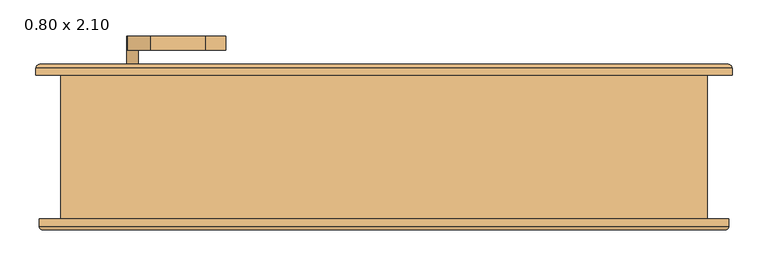
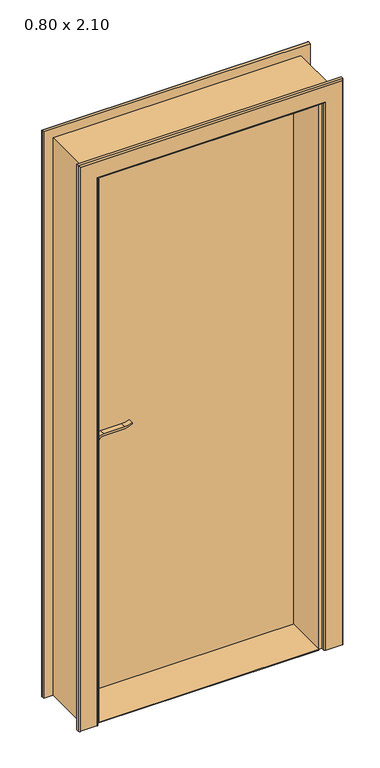
"""IFC4 building model written with IfcOpenShell, lengths in millimetres: door geometry, PORTA_DE_ABRIR_MADEIRA : 0.80 x 2.10."""

from ifc_helpers import new_model, si_unit, point, frame, frame_2d, origin, origin_with_axes, place, context, project, spatial, polyline, circle_curve, ellipse_curve, trimmed, segment, composite_curve, outline, extrude, faceted_brep, source, transform, mapped, element, save
from ifc_brep_helpers import plane_surface, cylinder_surface, advanced_brep


def door_0_80_x_2_10_3d2226a5(model_context):
    return source(origin(), model_context, "Body", "SolidModel", [
        extrude(outline(composite_curve([segment(trimmed(circle_curve(frame_2d((940.0, -350.0)), 15.0), [point((940.0, -335.0))], [point((940.0, -365.0))], False, "CARTESIAN"), True, "CONTINUOUS"), segment(trimmed(circle_curve(frame_2d((940.0, -350.0)), 15.0), [point((940.0, -365.0))], [point((940.0, -335.0))], False, "CARTESIAN"), True, "CONTINUOUS")], self_intersect=False)), frame((0.0, 40.0, 0.0), z_axis=(0.0, 1.0, 0.0), x_axis=(0.0, 0.0, 1.0)), (0.0, 0.0, 1.0), 10.0),
        extrude(outline(composite_curve([segment(trimmed(circle_curve(frame_2d((940.0, -350.0)), 15.0), [point((940.0, -335.0))], [point((940.0, -365.0))], False, "CARTESIAN"), True, "CONTINUOUS"), segment(trimmed(circle_curve(frame_2d((940.0, -350.0)), 15.0), [point((940.0, -365.0))], [point((940.0, -335.0))], False, "CARTESIAN"), True, "CONTINUOUS")], self_intersect=False)), frame((0.0, 105.0, 0.0), z_axis=(0.0, 1.0, 0.0), x_axis=(0.0, 0.0, 1.0)), (0.0, 0.0, 1.0), 10.0),
        extrude(outline(composite_curve([segment(trimmed(circle_curve(frame_2d((1000.0, -350.0)), 8.0), [point((1004.6523287, -356.5081363))], [point((1000.0, -342.0))], False, "CARTESIAN"), True, "CONTINUOUS"), segment(trimmed(circle_curve(frame_2d((994.8738613, -324.6138099)), 18.1261387), [point((1000.0, -342.0))], [point((1013.0, -324.6138099))], True, "CARTESIAN"), True, "CONTINUOUS"), segment(polyline([(1013.0, -324.6138099), (1013.0, -248.3564091)]), True, "CONTINUOUS"), segment(trimmed(circle_curve(frame_2d((1072.2709207, -251.9396612)), 59.3791355), [point((1013.0, -248.3564091))], [point((1022.2135558, -220.0))], False, "CARTESIAN"), True, "CONTINUOUS"), segment(polyline([(1022.2135558, -220.0), (1025.0, -220.0)]), True, "CONTINUOUS"), segment(trimmed(circle_curve(frame_2d((1103.2850638, -248.4227909)), 83.2850902), [point((1025.0, -220.0))], [point((1020.0, -248.3564091))], True, "CARTESIAN"), True, "CONTINUOUS"), segment(polyline([(1020.0, -248.3564091), (1020.0, -324.6325667)]), True, "CONTINUOUS"), segment(trimmed(circle_curve(frame_2d((982.7555521, -326.3324871)), 37.2832219), [point((1020.0, -324.6325667))], [point((1004.6523287, -356.5081363))], False, "CARTESIAN"), True, "CONTINUOUS")], self_intersect=False)), frame((0.0, 0.0, 0.0), z_axis=(0.0, 1.0, 0.0), x_axis=(0.0, 0.0, 1.0)), (0.0, 0.0, 1.0), 20.0),
        extrude(outline(composite_curve([segment(trimmed(circle_curve(frame_2d((994.8738682, -324.6138122)), 18.1261318), [point((999.9999903, -342.0))], [point((1013.0, -324.6138122))], True, "CARTESIAN"), True, "CONTINUOUS"), segment(polyline([(1013.0, -324.6138122), (1013.0, -248.3564091)]), True, "CONTINUOUS"), segment(trimmed(circle_curve(frame_2d((1072.2709207, -251.9396612)), 59.3791355), [point((1013.0, -248.3564091))], [point((1022.2135558, -220.0))], False, "CARTESIAN"), True, "CONTINUOUS"), segment(polyline([(1022.2135558, -220.0), (1025.0, -220.0)]), True, "CONTINUOUS"), segment(trimmed(circle_curve(frame_2d((1103.2850638, -248.4227909)), 83.2850902), [point((1025.0, -220.0))], [point((1020.0, -248.3564091))], True, "CARTESIAN"), True, "CONTINUOUS"), segment(polyline([(1020.0, -248.3564091), (1020.0, -324.6325667)]), True, "CONTINUOUS"), segment(trimmed(circle_curve(frame_2d((982.7555521, -326.3324871)), 37.2832219), [point((1020.0, -324.6325667))], [point((1004.6523287, -356.5081363))], False, "CARTESIAN"), True, "CONTINUOUS"), segment(trimmed(circle_curve(frame_2d((1000.0, -350.0)), 8.0), [point((1004.6523287, -356.5081363))], [point((999.9999903, -342.0))], False, "CARTESIAN"), True, "CONTINUOUS")], self_intersect=False)), frame((0.0, 135.0, 0.0), z_axis=(0.0, 1.0, 0.0), x_axis=(0.0, 0.0, 1.0)), (0.0, 0.0, 1.0), 20.0),
        extrude(outline(composite_curve([segment(trimmed(circle_curve(frame_2d((1000.0, -350.0)), 8.0), [point((1000.0, -342.0))], [point((1000.0, -358.0))], False, "CARTESIAN"), True, "CONTINUOUS"), segment(trimmed(circle_curve(frame_2d((1000.0, -350.0)), 8.0), [point((1000.0, -358.0))], [point((1000.0, -342.0))], False, "CARTESIAN"), True, "CONTINUOUS")], self_intersect=False)), frame((0.0, 20.0, 0.0), z_axis=(0.0, 1.0, 0.0), x_axis=(0.0, 0.0, 1.0)), (0.0, 0.0, 1.0), 30.0),
        extrude(outline(composite_curve([segment(trimmed(circle_curve(frame_2d((1000.0, -350.0)), 8.0), [point((1000.0, -342.0))], [point((1000.0, -358.0))], False, "CARTESIAN"), True, "CONTINUOUS"), segment(trimmed(circle_curve(frame_2d((1000.0, -350.0)), 8.0), [point((1000.0, -358.0))], [point((1000.0, -342.0))], False, "CARTESIAN"), True, "CONTINUOUS")], self_intersect=False)), frame((0.0, 105.0, 0.0), z_axis=(0.0, 1.0, 0.0), x_axis=(0.0, 0.0, 1.0)), (0.0, 0.0, 1.0), 30.0),
        extrude(outline(composite_curve([segment(trimmed(circle_curve(frame_2d((930.0, -350.0)), 25.0), [point((930.0, -375.0))], [point((930.0, -325.0))], False, "CARTESIAN"), True, "CONTINUOUS"), segment(polyline([(930.0, -325.0), (1000.0, -325.0)]), True, "CONTINUOUS"), segment(trimmed(circle_curve(frame_2d((1000.0, -350.0)), 25.0), [point((1000.0, -325.0))], [point((1000.0, -375.0))], False, "CARTESIAN"), True, "CONTINUOUS"), segment(polyline([(1000.0, -375.0), (930.0, -375.0)]), True, "CONTINUOUS")], self_intersect=False)), frame((0.0, 50.0, 0.0), z_axis=(0.0, 1.0, 0.0), x_axis=(0.0, 0.0, 1.0)), (0.0, 0.0, 1.0), 10.0),
        extrude(outline(composite_curve([segment(trimmed(circle_curve(frame_2d((930.0, -350.0)), 25.0), [point((930.0, -375.0))], [point((930.0, -325.0))], False, "CARTESIAN"), True, "CONTINUOUS"), segment(polyline([(930.0, -325.0), (1000.0, -325.0)]), True, "CONTINUOUS"), segment(trimmed(circle_curve(frame_2d((1000.0, -350.0)), 25.0), [point((1000.0, -325.0))], [point((1000.0, -375.0))], False, "CARTESIAN"), True, "CONTINUOUS"), segment(polyline([(1000.0, -375.0), (930.0, -375.0)]), True, "CONTINUOUS")], self_intersect=False)), frame((0.0, 95.0, 0.0), z_axis=(0.0, 1.0, 0.0), x_axis=(0.0, 0.0, 1.0)), (0.0, 0.0, 1.0), 10.0),
        faceted_brep([(-410.0, 60.0, 0.0), (-400.0, 60.0, 0.0), (-400.0, -100.0, 0.0), (-450.0, -100.0, 0.0), (-450.0, 100.0, 0.0), (-410.0, 100.0, 0.0), (-410.0, 100.0, 2100.0), (-410.0, 60.0, 2100.0), (-450.0, 100.0, 2140.0), (450.0, 100.0, 2140.0), (450.0, 100.0, 0.0), (410.0, 100.0, 0.0), (410.0, 100.0, 2100.0), (-450.0, -100.0, 2140.0), (-400.0, -100.0, 2090.0), (400.0, -100.0, 2090.0), (400.0, -100.0, 0.0), (450.0, -100.0, 0.0), (450.0, -100.0, 2140.0), (-400.0, 60.0, 2090.0), (410.0, 60.0, 2100.0), (410.0, 60.0, 0.0), (400.0, 60.0, 0.0), (400.0, 60.0, 2090.0)], [[[0, 1, 2, 3, 4, 5]], [[5, 6, 7, 0]], [[4, 8, 9, 10, 11, 12, 6, 5]], [[3, 13, 8, 4]], [[2, 14, 15, 16, 17, 18, 13, 3]], [[1, 19, 14, 2]], [[0, 7, 20, 21, 22, 23, 19, 1]], [[23, 22, 16, 15]], [[21, 11, 10, 17, 16, 22]], [[12, 11, 21, 20]], [[18, 17, 10, 9]], [[13, 18, 9, 8]], [[19, 23, 15, 14]], [[6, 12, 20, 7]]]),
        advanced_brep(
        [(-480.0, -100.3, 0.0), (-410.0, -100.3, 0.0), (-410.0, -110.3, 0.0), (-415.0, -115.3, 0.0), (-475.0, -115.3, 0.0), (-480.0, -110.3, 0.0), (-480.0, -110.3, 2170.0), (-480.0, -100.3, 2170.0), (-475.0, -115.3, 2165.0), (-415.0, -115.3, 2105.0), (415.0, -115.3, 2105.0), (415.0, -115.3, 0.0), (475.0, -115.3, 0.0), (475.0, -115.3, 2165.0), (-410.0, -110.3, 2100.0), (-410.0, -100.3, 2100.0), (480.0, -100.3, 2170.0), (480.0, -100.3, 0.0), (410.0, -100.3, 0.0), (410.0, -100.3, 2100.0), (480.0, -110.3, 0.0), (410.0, -110.3, 0.0), (410.0, -110.3, 2100.0), (480.0, -110.3, 2170.0)],
        [
            (0, 1),
            (1, 2),
            (2, 3, circle_curve(frame((-415.0, -110.3, 0.0), z_axis=(0.0, 0.0, -1.0), x_axis=(-1.0, 0.0, 0.0)), 5.0)),
            (3, 4),
            (4, 5, circle_curve(frame((-475.0, -110.3, 0.0), z_axis=(0.0, 0.0, -1.0), x_axis=(-1.0, 0.0, 0.0)), 5.0)),
            (5, 0),
            (5, 6),
            (6, 7),
            (7, 0),
            (4, 8),
            (8, 6, ellipse_curve(frame((-475.0, -110.3, 2165.0), z_axis=(-0.7071067811865475, 0.0, -0.7071067811865475), x_axis=(0.7071067811865474, 0.0, -0.7071067811865476)), 7.0710678, 5.0)),
            (3, 9),
            (9, 10),
            (10, 11),
            (11, 12),
            (12, 13),
            (13, 8),
            (2, 14),
            (14, 9, ellipse_curve(frame((-415.0, -110.3, 2105.0), z_axis=(-0.7071067811865475, 0.0, -0.7071067811865475), x_axis=(0.7071067811865474, 0.0, -0.7071067811865476)), 7.0710678, 5.0)),
            (1, 15),
            (15, 14),
            (7, 16),
            (16, 17),
            (17, 18),
            (18, 19),
            (19, 15),
            (17, 20),
            (20, 12, circle_curve(frame((475.0, -110.3, 0.0), z_axis=(0.0, 0.0, -1.0), x_axis=(1.0, 0.0, 0.0)), 5.0)),
            (11, 21, circle_curve(frame((415.0, -110.3, 0.0), z_axis=(0.0, 0.0, -1.0), x_axis=(1.0, 0.0, 0.0)), 5.0)),
            (21, 18),
            (21, 22),
            (22, 19),
            (10, 22, ellipse_curve(frame((415.0, -110.3, 2105.0), z_axis=(0.7071067811865475, 0.0, -0.7071067811865475), x_axis=(0.7071067811865474, 0.0, 0.7071067811865476)), 7.0710678, 5.0)),
            (20, 23),
            (23, 13, ellipse_curve(frame((475.0, -110.3, 2165.0), z_axis=(0.7071067811865475, 0.0, -0.7071067811865475), x_axis=(0.7071067811865474, 0.0, 0.7071067811865476)), 7.0710678, 5.0)),
            (16, 23),
            (6, 23),
            (22, 14),
        ],
        [
            plane_surface(frame((-450.0, 100.0, 0.0), z_axis=(0.0, 0.0, -1.0), x_axis=(0.0, 1.0, 0.0))),
            plane_surface(frame((-480.0, -100.3, 0.0), z_axis=(-1.0, 0.0, 0.0), x_axis=(0.0, 0.0, 1.0))),
            cylinder_surface(frame((-475.0, -110.3, 0.0), z_axis=(0.0, 0.0, -1.0), x_axis=(-1.0, 0.0, 0.0)), 5.0),
            plane_surface(frame((-475.0, -115.3, 0.0), z_axis=(0.0, -1.0, 0.0), x_axis=(0.0, 0.0, 1.0))),
            cylinder_surface(frame((-415.0, -110.3, 0.0), z_axis=(0.0, 0.0, -1.0), x_axis=(-1.0, 0.0, 0.0)), 5.0),
            plane_surface(frame((-410.0, -110.3, 0.0), z_axis=(1.0, 0.0, 0.0), x_axis=(0.0, 0.0, 1.0))),
            plane_surface(frame((-410.0, -100.3, 0.0), z_axis=(0.0, 1.0, 0.0), x_axis=(0.0, 0.0, 1.0))),
            plane_surface(frame((450.0, 100.0, 0.0), z_axis=(0.0, 0.0, -1.0), x_axis=(0.0, 1.0, 0.0))),
            plane_surface(frame((410.0, -110.3, 2100.0), z_axis=(-1.0, 0.0, 0.0), x_axis=(0.0, 0.0, -1.0))),
            cylinder_surface(frame((415.0, -110.3, 2140.0), z_axis=(0.0, 0.0, 1.0), x_axis=(1.0, 0.0, 0.0)), 5.0),
            cylinder_surface(frame((475.0, -110.3, 2140.0), z_axis=(0.0, 0.0, 1.0), x_axis=(1.0, 0.0, 0.0)), 5.0),
            plane_surface(frame((480.0, -100.3, 2170.0), z_axis=(1.0, 0.0, 0.0), x_axis=(0.0, 0.0, -1.0))),
            plane_surface(frame((-480.0, -100.3, 2170.0), z_axis=(0.0, 0.0, 1.0), x_axis=(1.0, 0.0, 0.0))),
            plane_surface(frame((-410.0, -110.3, 2100.0), z_axis=(0.0, 0.0, -1.0), x_axis=(1.0, 0.0, 0.0))),
            cylinder_surface(frame((-450.0, -110.3, 2165.0), z_axis=(-1.0, 0.0, 0.0), x_axis=(0.0, 0.0, 1.0)), 5.0),
            cylinder_surface(frame((-450.0, -110.3, 2105.0), z_axis=(-1.0, 0.0, 0.0), x_axis=(0.0, 0.0, 1.0)), 5.0),
        ],
        [
            (0, [[1, 2, 3, 4, 5, 6]]),
            (1, [[7, 8, 9, -6]]),
            (2, [[10, 11, -7, -5]]),
            (3, [[12, 13, 14, 15, 16, 17, -10, -4]]),
            (4, [[18, 19, -12, -3]]),
            (5, [[20, 21, -18, -2]]),
            (6, [[-9, 22, 23, 24, 25, 26, -20, -1]]),
            (7, [[27, 28, -15, 29, 30, -24]]),
            (8, [[-25, -30, 31, 32]]),
            (9, [[-31, -29, -14, 33]]),
            (10, [[-16, -28, 34, 35]]),
            (11, [[-34, -27, -23, 36]]),
            (12, [[37, -36, -22, -8]]),
            (13, [[-26, -32, 38, -21]]),
            (14, [[-17, -35, -37, -11]]),
            (15, [[-38, -33, -13, -19]]),
        ],
    ),
        advanced_brep(
        [(-479.3155593, 115.2647517, 0.0), (-419.3155593, 115.2647517, 0.0), (-414.3155593, 110.2647517, 0.0), (-414.3155593, 100.2647517, 0.0), (-484.3155593, 100.2647517, 0.0), (-484.3155593, 110.2647517, 0.0), (-484.3155593, 110.2647517, 2174.3155593), (-479.3155593, 115.2647517, 2169.3155593), (-484.3155593, 100.2647517, 2174.3155593), (-414.3155593, 100.2647517, 2104.3155593), (414.3155593, 100.2647517, 2104.3155593), (414.3155593, 100.2647517, 0.0), (484.3155593, 100.2647517, 0.0), (484.3155593, 100.2647517, 2174.3155593), (-414.3155593, 110.2647517, 2104.3155593), (-419.3155593, 115.2647517, 2109.3155593), (479.3155593, 115.2647517, 2169.3155593), (479.3155593, 115.2647517, 0.0), (419.3155593, 115.2647517, 0.0), (419.3155593, 115.2647517, 2109.3155593), (484.3155593, 110.2647517, 0.0), (414.3155593, 110.2647517, 0.0), (414.3155593, 110.2647517, 2104.3155593), (484.3155593, 110.2647517, 2174.3155593)],
        [
            (0, 1),
            (1, 2, circle_curve(frame((-419.3155593, 110.2647517, 0.0), z_axis=(0.0, 0.0, -1.0), x_axis=(-1.0, 0.0, 0.0)), 5.0)),
            (2, 3),
            (3, 4),
            (4, 5),
            (5, 0, circle_curve(frame((-479.3155593, 110.2647517, 0.0), z_axis=(0.0, 0.0, -1.0), x_axis=(-1.0, 0.0, 0.0)), 5.0)),
            (5, 6),
            (6, 7, ellipse_curve(frame((-479.3155593, 110.2647517, 2169.3155593), z_axis=(-0.7071067811865475, 0.0, -0.7071067811865475), x_axis=(0.7071067811865474, 0.0, -0.7071067811865476)), 7.0710678, 5.0)),
            (7, 0),
            (4, 8),
            (8, 6),
            (3, 9),
            (9, 10),
            (10, 11),
            (11, 12),
            (12, 13),
            (13, 8),
            (2, 14),
            (14, 9),
            (1, 15),
            (15, 14, ellipse_curve(frame((-419.3155593, 110.2647517, 2109.3155593), z_axis=(-0.7071067811865475, 0.0, -0.7071067811865475), x_axis=(0.7071067811865474, 0.0, -0.7071067811865476)), 7.0710678, 5.0)),
            (7, 16),
            (16, 17),
            (17, 18),
            (18, 19),
            (19, 15),
            (17, 20, circle_curve(frame((479.3155593, 110.2647517, 0.0), z_axis=(0.0, 0.0, -1.0), x_axis=(1.0, 0.0, 0.0)), 5.0)),
            (20, 12),
            (11, 21),
            (21, 18, circle_curve(frame((419.3155593, 110.2647517, 0.0), z_axis=(0.0, 0.0, -1.0), x_axis=(1.0, 0.0, 0.0)), 5.0)),
            (21, 22),
            (22, 19, ellipse_curve(frame((419.3155593, 110.2647517, 2109.3155593), z_axis=(0.7071067811865475, 0.0, -0.7071067811865475), x_axis=(0.7071067811865474, 0.0, 0.7071067811865476)), 7.0710678, 5.0)),
            (10, 22),
            (20, 23),
            (23, 13),
            (16, 23, ellipse_curve(frame((479.3155593, 110.2647517, 2169.3155593), z_axis=(0.7071067811865475, 0.0, -0.7071067811865475), x_axis=(0.7071067811865474, 0.0, 0.7071067811865476)), 7.0710678, 5.0)),
            (23, 6),
            (14, 22),
        ],
        [
            plane_surface(frame((-450.0, 100.0, 0.0), z_axis=(0.0, 0.0, -1.0), x_axis=(0.0, 1.0, 0.0))),
            cylinder_surface(frame((-479.3155593, 110.2647517, 0.0), z_axis=(0.0, 0.0, -1.0), x_axis=(-1.0, 0.0, 0.0)), 5.0),
            plane_surface(frame((-484.3155593, 110.2647517, 0.0), z_axis=(-1.0, 0.0, 0.0), x_axis=(0.0, 0.0, 1.0))),
            plane_surface(frame((-484.3155593, 100.2647517, 0.0), z_axis=(0.0, -1.0, 0.0), x_axis=(0.0, 0.0, 1.0))),
            plane_surface(frame((-414.3155593, 100.2647517, 0.0), z_axis=(1.0, 0.0, 0.0), x_axis=(0.0, 0.0, 1.0))),
            cylinder_surface(frame((-419.3155593, 110.2647517, 0.0), z_axis=(0.0, 0.0, -1.0), x_axis=(-1.0, 0.0, 0.0)), 5.0),
            plane_surface(frame((-419.3155593, 115.2647517, 0.0), z_axis=(0.0, 1.0, 0.0), x_axis=(0.0, 0.0, 1.0))),
            plane_surface(frame((450.0, 100.0, 0.0), z_axis=(0.0, 0.0, -1.0), x_axis=(0.0, 1.0, 0.0))),
            cylinder_surface(frame((419.3155593, 110.2647517, 2140.0), z_axis=(0.0, 0.0, 1.0), x_axis=(1.0, 0.0, 0.0)), 5.0),
            plane_surface(frame((414.3155593, 100.2647517, 2104.3155593), z_axis=(-1.0, 0.0, 0.0), x_axis=(0.0, 0.0, -1.0))),
            plane_surface(frame((484.3155593, 110.2647517, 2174.3155593), z_axis=(1.0, 0.0, 0.0), x_axis=(0.0, 0.0, -1.0))),
            cylinder_surface(frame((479.3155593, 110.2647517, 2140.0), z_axis=(0.0, 0.0, 1.0), x_axis=(1.0, 0.0, 0.0)), 5.0),
            plane_surface(frame((-484.3155593, 110.2647517, 2174.3155593), z_axis=(0.0, 0.0, 1.0), x_axis=(1.0, 0.0, 0.0))),
            plane_surface(frame((-414.3155593, 100.2647517, 2104.3155593), z_axis=(0.0, 0.0, -1.0), x_axis=(1.0, 0.0, 0.0))),
            cylinder_surface(frame((-450.0, 110.2647517, 2169.3155593), z_axis=(-1.0, 0.0, 0.0), x_axis=(0.0, 0.0, 1.0)), 5.0),
            cylinder_surface(frame((-450.0, 110.2647517, 2109.3155593), z_axis=(-1.0, 0.0, 0.0), x_axis=(0.0, 0.0, 1.0)), 5.0),
        ],
        [
            (0, [[1, 2, 3, 4, 5, 6]]),
            (1, [[7, 8, 9, -6]]),
            (2, [[10, 11, -7, -5]]),
            (3, [[12, 13, 14, 15, 16, 17, -10, -4]]),
            (4, [[18, 19, -12, -3]]),
            (5, [[20, 21, -18, -2]]),
            (6, [[-9, 22, 23, 24, 25, 26, -20, -1]]),
            (7, [[27, 28, -15, 29, 30, -24]]),
            (8, [[-25, -30, 31, 32]]),
            (9, [[-31, -29, -14, 33]]),
            (10, [[-16, -28, 34, 35]]),
            (11, [[-34, -27, -23, 36]]),
            (12, [[-17, -35, 37, -11]]),
            (13, [[38, -33, -13, -19]]),
            (14, [[-37, -36, -22, -8]]),
            (15, [[-26, -32, -38, -21]]),
        ],
    ),
        extrude(outline(polyline([(410.0, 95.0), (410.0, 60.0), (-410.0, 60.0), (-410.0, 95.0), (410.0, 95.0)])), origin_with_axes(), (0.0, 0.0, 1.0), 2100.0),
        extrude(outline(polyline([(-400.0, 35.0), (-410.0, 35.0), (-410.0, 100.0), (410.0, 100.0), (410.0, 35.0), (400.0, 35.0), (400.0, -100.0), (-400.0, -100.0), (-400.0, 35.0)])), frame((0.0, 0.0, -3.0), z_axis=(0.0, 0.0, 1.0), x_axis=(1.0, 0.0, 0.0)), (0.0, 0.0, 1.0), 3.1),
    ])


if __name__ == "__main__":
    model = new_model("IFC4")
    model_context = context("Model", 3, world=origin())
    ifc_project = project(units=[si_unit("LENGTHUNIT", "METRE", prefix="MILLI")], contexts=[model_context])
    site = spatial("IfcSite", under=ifc_project)
    building = spatial("IfcBuilding", under=site)
    placement = place(None, origin())
    door_0_80_x_2_10_shape = door_0_80_x_2_10_3d2226a5(model_context)
    element("IfcDoor", 1, ObjectType="PORTA_DE_ABRIR_MADEIRA : 0.80 x 2.10", at=placement, inside=building, context=model_context, shape_type="MappedRepresentation", body=[
        mapped(door_0_80_x_2_10_shape, transform((0.0, 0.0, 0.0), x_axis=(1.0, 0.0, 0.0), y_axis=(0.0, 1.0, 0.0), z_axis=(0.0, 0.0, 1.0))),
    ])
    save(model, "model.ifc")

# Revit data of these elements
# Type "PORTA_DE_ABRIR_MADEIRA : 0.80 x 2.10"
#   Type Mark = "P2"
#   Analytic Construction = "<Nenhum>"
#   Rough Width = 0.90 m
#   Projeção da estrutura externa = 0.50 m
#   Projeção da estrutura interna = 0.025 m
#   Largura da estrutura = 0.075 m
#   Rough Height = 2.15 m
#   Height = 2.10 m
#   Width = 0.80 m
#   Soleira [instance default] = no
#   Material do batente = .BATENTE E GUARNIÇÃO
#   Material da maçaneta = .AÇO INOXIDÁVEL ESCOVADO
#   Material da folha da porta = .FOLHA DA PORTA
#   Material da Soleira [instance default] = none
#   Function = (empty or 0)
#   Wall Closure = (empty or 0)
# Element 1 (IfcDoor, "PORTA_DE_ABRIR_MADEIRA : 0.80 x 2.10")
#   Soleira = yes
#   Material da Soleira = .GRANITO BRANCO ITAUNAS
#   Materials on its faces: ".AÇO INOXIDÁVEL ESCOVADO", ".BATENTE E GUARNIÇÃO", ".GRANITO BRANCO ITAUNAS", ".FOLHA DA PORTA"
# Materials
#   ".BATENTE E GUARNIÇÃO": class "Madeira", colour RGB 215 186 156, transparency 0, Cost = 0
#   ".AÇO INOXIDÁVEL ESCOVADO": class "Metal", colour RGB 189 187 185, transparency 0, Description = "Stainless Steel 18/8, brushed finish", Cost = 0
#   ".FOLHA DA PORTA": class "Madeira", colour RGB 148 119 91, transparency 0, Cost = 0
#   ".GRANITO BRANCO ITAUNAS": class ".CC_PEDRA REVEST.", colour RGB 202 195 174, transparency 0, Description = "Revestimento em granito", Cost = 0
